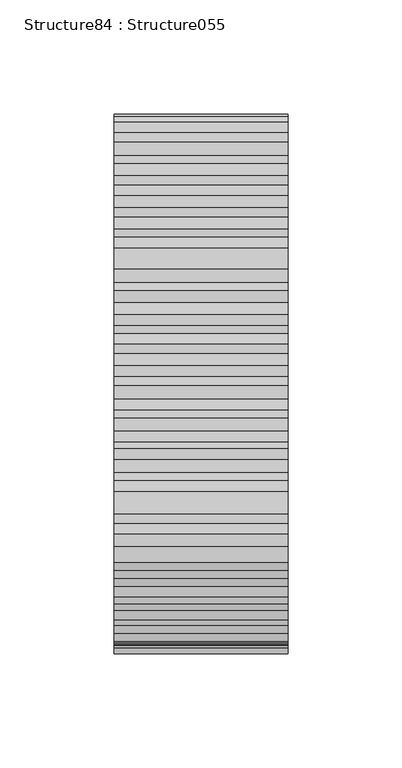
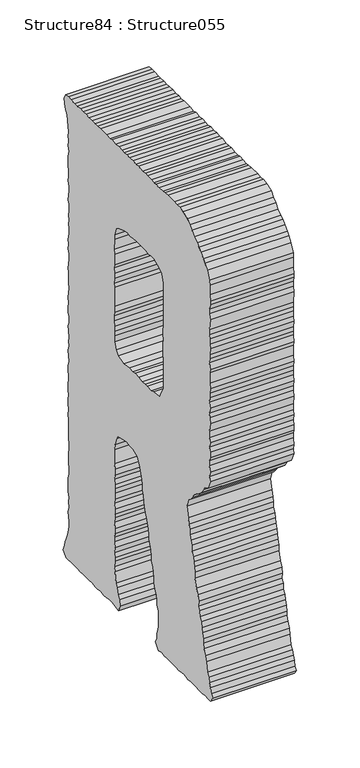
"""IFC4 building model written with IfcOpenShell, lengths in millimetres: proxy geometry, Structure84 : Structure055."""

from ifc_helpers import new_model, si_unit, frame, origin, place, context, project, spatial, polyline, outline, extrude, source, transform, mapped, element, save


def structure84_structure055_91e5d643(model_context):
    return source(origin(), model_context, "Body", "SweptSolid", [
        extrude(outline(polyline([(279847.3138798, 3899.7046941), (279847.8979559, 3903.2059411), (279847.8979559, 3907.888177), (279846.7233854, 3918.4480792), (279847.8979559, 3923.1319197), (279847.8979559, 3927.8077372), (279846.7233854, 3932.4899731), (279846.7233854, 3936.0345445), (279847.3138798, 3941.8753048), (279847.3138798, 3951.2606365), (279847.8979559, 3955.360401), (279851.4136443, 3962.9774586), (279854.9309374, 3967.6789497), (279857.2640323, 3970.5768654), (279861.3734244, 3974.1214368), (279864.2970138, 3977.6194746), (279867.2414631, 3979.9621971), (279871.915676, 3982.8793681), (279875.4313644, 3987.0048063), (279878.9566805, 3989.9460463), (279882.4771827, 3994.0233463), (279889.5005366, 3996.390138), (279894.7668486, 3997.5486624), (279899.4603167, 3996.9645864), (279903.5584766, 3997.5486624), (279913.5182567, 3997.5486624), (279918.2117249, 3996.9645864), (279921.7193903, 3996.390138), (279927.5874289, 3996.390138), (279932.2616418, 3996.9645864), (279935.2060911, 3996.390138), (279939.8786994, 3996.390138), (279945.746738, 3996.9645864), (279949.2640311, 3996.9645864), (279953.9574992, 3996.390138), (279959.8078872, 3997.5486624), (279963.9172793, 3996.9645864), (279968.5995152, 3997.5486624), (279973.8658272, 3996.9645864), (279977.9655917, 3997.5486624), (279982.6590598, 3996.390138), (279986.1763529, 3996.9645864), (279990.8682164, 3997.5486624), (279996.136133, 3996.390138), (280001.410468, 3997.5486624), (280004.927761, 3996.390138), (280010.778149, 3996.9645864), (280020.1618761, 3996.9645864), (280024.8457166, 3996.390138), (280028.3614051, 3996.9645864), (280033.6309262, 3996.390138), (280037.7403183, 3996.9645864), (280043.0146533, 3996.9645864), (280047.6968892, 3996.390138), (280051.7886307, 3996.9645864), (280057.0725933, 3996.390138), (280060.583468, 3996.390138), (280066.4482974, 3996.9645864), (280070.5400388, 3996.9645864), (280075.233507, 3996.390138), (280077.582648, 3991.6806238), (280077.0017811, 3986.4046842), (280075.233507, 3981.7208437), (280072.892389, 3978.2035506), (280071.7178185, 3973.5197101), (280070.5400388, 3963.5615346), (280071.1337425, 3959.4617701), (280070.5400388, 3954.7506513), (280071.1337425, 3949.4923624), (280069.9655904, 3944.8165449), (280071.1337425, 3939.5325823), (280071.1337425, 3930.1745289), (280070.5400388, 3926.6492128), (280070.5400388, 3920.7908018), (280071.1337425, 3916.0909152), (280069.9655904, 3911.4054701), (280069.9655904, 3906.7328618), (280070.5400388, 3903.2059411), (280071.1337425, 3897.3475301), (280069.9655904, 3893.822214), (280069.9655904, 3887.9621984), (280070.5400388, 3883.2863809), (280069.9655904, 3878.5784713), (280070.5400388, 3875.0772243), (280069.9655904, 3870.4030114), (280069.9655904, 3865.7015202), (280071.1337425, 3859.8591552), (280070.5400388, 3855.7353217), (280071.1337425, 3850.4754282), (280069.9655904, 3846.3772683), (280069.9655904, 3841.0900965), (280070.5400388, 3836.9919366), (280071.1337425, 3831.732043), (280070.5400388, 3828.2163546), (280070.5400388, 3818.2309008), (280069.9655904, 3812.9726119), (280070.5400388, 3809.4729695), (280071.1337425, 3803.5872802), (280070.5400388, 3798.9050443), (280071.1337425, 3794.8309535), (280071.1337425, 3789.5293402), (280069.9655904, 3786.0280932), (280069.9655904, 3780.1616592), (280071.1337425, 3776.6427615), (280070.5400388, 3771.9605256), (280069.9655904, 3766.1021146), (280070.5400388, 3761.418274), (280069.9655904, 3757.8753073), (280071.1337425, 3752.6170184), (280070.5400388, 3747.9428055), (280069.9655904, 3742.6748889), (280071.1337425, 3738.5574738), (280071.1337425, 3733.2991849), (280070.5400388, 3729.1737467), (280070.5400388, 3725.0996559), (280071.1337425, 3720.4158154), (280071.1337425, 3714.5301261), (280070.5400388, 3709.8559132), (280071.1337425, 3706.3289925), (280071.1337425, 3701.6547796), (280070.5400388, 3695.786741), (280071.1337425, 3691.0868544), (280070.5400388, 3686.4030139), (280070.5400388, 3668.2437048), (280069.9655904, 3663.5598643), (280069.9655904, 3658.8840468), (280070.5400388, 3654.1841602), (280070.5400388, 3645.4262289), (280069.9655904, 3639.5405396), (280069.9655904, 3634.856699), (280071.1337425, 3630.1824862), (280071.1337425, 3616.69739), (280069.9655904, 3612.0135494), (280070.5400388, 3607.8961343), (280069.9655904, 3602.0280957), (280071.1337425, 3597.9540049), (280069.9655904, 3588.5702778), (280069.9655904, 3583.8864372), (280072.308313, 3574.5107332), (280073.4844881, 3570.9854171), (280075.8159784, 3565.7094775), (280077.0017811, 3561.6257591), (280078.7508, 3556.3417965), (280074.6414079, 3551.0658569), (280070.5400388, 3551.0658569), (280066.4482974, 3551.6675836), (280056.4820989, 3551.6675836), (280052.3823344, 3551.0658569), (280047.6968892, 3551.6675836), (280037.7403183, 3551.6675836), (280033.0468502, 3552.242032), (280028.9551087, 3551.0658569), (280024.2632452, 3551.0658569), (280020.1618761, 3551.6675836), (280015.4684079, 3551.0658569), (280010.2037006, 3551.6675836), (280006.1023315, 3552.242032), (280001.9929394, 3552.242032), (279997.3107035, 3551.0658569), (279991.4506879, 3550.4833855), (279989.0999423, 3556.3417965), (279990.2761174, 3561.6257591), (279992.6172353, 3565.1254015), (279993.7934104, 3570.9854171), (279995.5424293, 3574.5107332), (279996.7169998, 3585.0706354), (279997.8947795, 3589.1527492), (279997.3107035, 3594.4286888), (279997.3107035, 3597.9540049), (279997.8947795, 3602.6298224), (279996.7169998, 3607.8961343), (279997.8947795, 3613.1720739), (279997.8947795, 3617.2718384), (279996.7169998, 3621.3732075), (279996.7169998, 3626.0554434), (279997.8947795, 3631.915459), (279997.3107035, 3636.6153456), (279996.7169998, 3640.114988), (279996.7169998, 3644.8245022), (279997.8947795, 3650.1004418), (279997.3107035, 3654.1841602), (279997.3107035, 3660.0682449), (279996.7169998, 3664.7440624), (279997.3107035, 3668.2437048), (279997.8947795, 3672.9435914), (279996.7169998, 3677.6274319), (279996.7169998, 3683.4858429), (279997.8947795, 3688.1873341), (279997.8947795, 3701.6547796), (279996.7169998, 3706.9130685), (279994.9679809, 3713.9556777), (279992.0347639, 3717.4729707), (279983.8336303, 3719.8140887), (279977.9655917, 3720.9726131), (279974.4579262, 3719.8140887), (279968.5995152, 3719.8140887), (279961.5745568, 3716.8985223), (279957.4731877, 3709.2718371), (279956.2986172, 3703.4134261), (279954.5319476, 3698.711935), (279953.3637955, 3695.2122926), (279953.3637955, 3689.3458585), (279952.1892251, 3685.2444894), (279951.01305, 3679.9701544), (279950.4321831, 3675.8687854), (279948.6815596, 3670.5848228), (279947.4957569, 3667.0851803), (279945.746738, 3662.3836892), (279944.5721675, 3657.7014533), (279943.3959924, 3652.4431643), (279943.3959924, 3648.3161216), (279942.229445, 3644.2420307), (279940.472403, 3639.5405396), (279939.8786994, 3634.856699), (279939.2978325, 3629.5984101), (279936.95511, 3625.472972), (279936.3710339, 3620.7971545), (279935.7805395, 3616.0972679), (279935.2060911, 3611.4134274), (279934.0283114, 3606.1551384), (279931.6791704, 3602.0280957), (279931.104722, 3596.7698067), (279930.5126229, 3592.6700423), (279928.1634819, 3588.5702778), (279928.1634819, 3583.2863152), (279928.1634819, 3573.9266571), (279929.3380524, 3570.4109687), (279930.5126229, 3565.1254015), (279931.104722, 3560.441561), (279932.8537409, 3556.3417965), (279928.1634819, 3550.4833855), (279923.4876644, 3551.6675836), (279919.3782723, 3550.4833855), (279915.2769032, 3551.0658569), (279901.7934117, 3551.0658569), (279895.9446283, 3550.4833855), (279891.2511601, 3551.6675836), (279887.7418901, 3551.6675836), (279881.8834791, 3550.4833855), (279877.7837146, 3551.6675836), (279868.990482, 3551.6675836), (279864.2970138, 3551.0658569), (279859.0307019, 3551.0658569), (279854.3404429, 3551.6675836), (279850.8215453, 3551.0658569), (279846.1393093, 3551.6675836), (279842.6220163, 3556.3417965), (279844.9711573, 3559.2669905), (279846.1393093, 3564.54293), (279847.8979559, 3568.0682461), (279849.0709217, 3572.7440636), (279851.4136443, 3576.2693797), (279853.1626632, 3585.0706354), (279854.3404429, 3590.3289243), (279856.6799563, 3595.5872132), (279857.8561314, 3600.2967274), (279857.8561314, 3604.3964919), (279859.0307019, 3609.6547808), (279860.2052723, 3613.772196), (279860.7813254, 3619.0385079), (279863.1320709, 3622.555801), (279863.7225654, 3627.8397636), (279865.4747935, 3631.3410106), (279864.8810898, 3636.6153456), (279866.0556603, 3641.8832621), (279868.3983829, 3646.557475), (279870.7491285, 3654.7842823), (279870.7491285, 3660.6250426), (279871.915676, 3665.3265338), (279872.507775, 3670.0007467), (279873.6727179, 3674.1277895), (279875.4313644, 3678.2018803), (279876.0154404, 3683.4858429), (279877.1900109, 3687.587212), (279878.9566805, 3691.6869765), (279878.9566805, 3696.9709391), (279880.1248326, 3701.0723082), (279881.29138, 3706.9130685), (279883.632498, 3716.2887726), (279881.29138, 3723.9154578), (279878.366186, 3726.2742264), (279875.4313644, 3729.7738688), (279871.915676, 3734.47536), (279867.8143069, 3737.9750024), (279864.8810898, 3739.7416719), (279860.7813254, 3743.2332913), (279857.8561314, 3747.9428055), (279854.9309374, 3751.4424479), (279850.8215453, 3753.8012165), (279846.7233854, 3762.5848215), (279847.8979559, 3766.684586), (279846.7233854, 3771.3860772), (279847.8979559, 3777.2444882), (279847.8979559, 3781.9299333), (279846.7233854, 3785.4456218), (279846.7233854, 3790.7039107), (279847.8979559, 3794.8309535), (279846.7233854, 3800.0876378), (279847.8979559, 3804.1890069), (279847.8979559, 3810.0474179), (279846.7233854, 3818.2309008), (279847.3138798, 3823.5341187), (279847.8979559, 3827.6162325), (279846.7233854, 3832.8921721), (279847.8979559, 3838.1761347), (279847.3138798, 3842.8583706), (279847.3138798, 3846.9757858), (279846.7233854, 3851.6612309), (279847.3138798, 3856.9179152), (279847.3138798, 3866.8776953), (279846.7233854, 3870.4030114), (279847.8979559, 3876.263027), (279847.3138798, 3880.3627915), (279847.3138798, 3884.4609514), (279846.7233854, 3890.320967), (279847.3138798, 3894.4030808), (279847.3138798, 3899.7046941)]), holes=[polyline([(279974.4579262, 3794.8309535), (279982.6590598, 3793.6451507), (279991.4506879, 3795.960595), (279994.3758819, 3800.0876378), (279997.3107035, 3805.9476534), (279996.7169998, 3811.7884138), (279996.7169998, 3816.4883003), (279997.3107035, 3820.5896694), (279997.8947795, 3825.849563), (279997.8947795, 3830.5574726), (279996.7169998, 3834.6588416), (279997.3107035, 3839.9331766), (279997.3107035, 3858.1021133), (279997.8947795, 3861.6178018), (279996.7169998, 3867.4601667), (279997.3107035, 3871.5599312), (279997.8947795, 3876.8438938), (279996.7169998, 3880.3627915), (279996.7169998, 3890.320967), (279997.8947795, 3894.4030808), (279996.7169998, 3904.9645876), (279996.7169998, 3909.0627475), (279994.3758819, 3916.0909152), (279990.8682164, 3918.4480792), (279982.6590598, 3921.3748778), (279977.9655917, 3922.5494483), (279973.2833558, 3921.3748778), (279969.7676673, 3921.9733953), (279963.9172793, 3922.5494483), (279949.2640311, 3922.5494483), (279944.5721675, 3921.3748778), (279941.0645021, 3922.5494483), (279936.3710339, 3922.5494483), (279927.5874289, 3919.0321552), (279924.0717405, 3915.5068392), (279921.1369189, 3908.46423), (279921.7193903, 3904.3901392), (279921.1369189, 3900.2887701), (279921.1369189, 3895.0048075), (279921.7193903, 3890.905043), (279921.1369189, 3885.6210804), (279921.7193903, 3880.9452629), (279921.7193903, 3876.8438938), (279921.1369189, 3871.5599312), (279921.1369189, 3867.4601667), (279922.313094, 3862.2018778), (279922.313094, 3858.1021133), (279921.7193903, 3854.0007442), (279922.313094, 3849.3008577), (279922.313094, 3839.9331766), (279921.7193903, 3834.0474873), (279921.7193903, 3829.374879), (279921.1369189, 3825.2911606), (279921.1369189, 3820.015221), (279921.7193903, 3816.4883003), (279921.7193903, 3810.6298893), (279921.1369189, 3806.5317294), (279925.2366833, 3800.0876378), (279926.9953299, 3795.960595), (279935.7805395, 3794.8309535), (279939.8786994, 3793.6451507), (279945.746738, 3794.2292268), (279949.2640311, 3794.2292268), (279953.9574992, 3793.6451507), (279959.2238112, 3794.8309535), (279965.0918498, 3794.8309535), (279968.5995152, 3794.2292268), (279974.4579262, 3794.8309535)])]), frame((-59031.6926606, 0.0, 0.0), z_axis=(1.0, 0.0, 0.0), x_axis=(0.0, 1.0, 0.0)), (0.0, 0.0, 1.0), 76.2),
    ])


if __name__ == "__main__":
    model = new_model("IFC4")
    model_context = context("Model", 3, world=origin())
    ifc_project = project(units=[si_unit("LENGTHUNIT", "METRE", prefix="MILLI")], contexts=[model_context])
    site = spatial("IfcSite", under=ifc_project)
    building = spatial("IfcBuilding", under=site)
    placement = place(None, origin())
    structure84_structure055_shape = structure84_structure055_91e5d643(model_context)
    element("IfcBuildingElementProxy", 1, Name="Structure84 : Structure055", ObjectType="Structure84 : Structure055", at=placement, inside=building, context=model_context, shape_type="MappedRepresentation", body=[
        mapped(structure84_structure055_shape, transform((0.0, 0.0, 0.0), x_axis=(1.0, 0.0, 0.0), y_axis=(0.0, 1.0, 0.0), z_axis=(0.0, 0.0, 1.0))),
    ])
    save(model, "model.ifc")

# Revit data of these elements
# Type "Structure84 : Structure055"
#   NameOverride = "Structure055"
# Element 1 (IfcBuildingElementProxy, "Structure84 : Structure055")
#   Materials on its faces: "BRUSHED ALUM. LETTERING"
# Materials
#   "BRUSHED ALUM. LETTERING": class "Unassigned", colour RGB 169 181 186, transparency 0, Cost = 0
